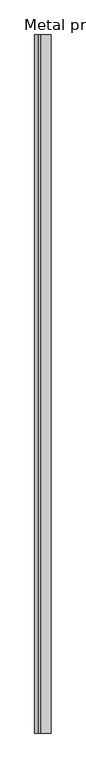
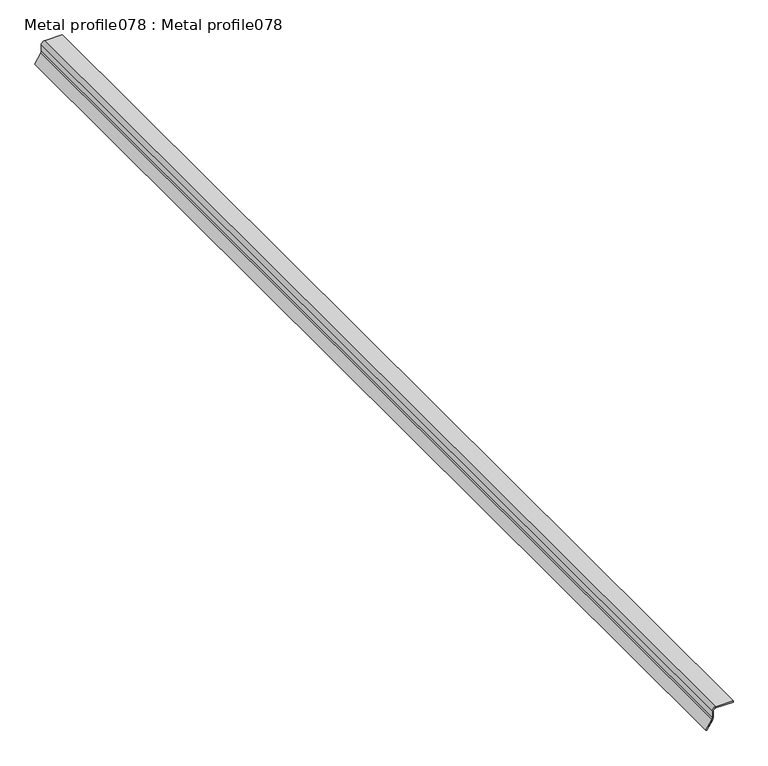
"""IFC4 building model written with IfcOpenShell, lengths in millimetres: proxy geometry, Metal profile078 : Metal profile078."""

from ifc_helpers import new_model, si_unit, point, frame, frame_2d, origin, place, context, project, spatial, polyline, circle_curve, trimmed, segment, composite_curve, outline, extrude, source, transform, mapped, element, save


def metal_profile078_metal_profile078_5d4c4150(model_context):
    return source(origin(), model_context, "Body", "SweptSolid", [
        extrude(outline(composite_curve([segment(polyline([(40166.609375, -9373.5329986), (40168.609375, -9373.5329986), (40168.609375, -9403.2796783)]), True, "CONTINUOUS"), segment(trimmed(circle_curve(frame_2d((40162.259375, -9403.2796783)), 6.35), [point((40168.609375, -9403.2796783))], [point((40162.259375, -9409.6296783))], False, "CARTESIAN"), True, "CONTINUOUS"), segment(polyline([(40162.259375, -9409.6296783), (40151.208717, -9409.6296783)]), True, "CONTINUOUS"), segment(trimmed(circle_curve(frame_2d((40151.208717, -9415.9796783)), 6.35), [point((40151.208717, -9409.6296783))], [point((40147.8972413, -9410.5615025))], True, "CARTESIAN"), True, "CONTINUOUS"), segment(polyline([(40147.8972413, -9410.5615025), (40131.8632813, -9420.3611236), (40130.8202968, -9418.6546115), (40146.8542568, -9408.8549905)]), True, "CONTINUOUS"), segment(trimmed(circle_curve(frame_2d((40151.208717, -9415.9796783)), 8.35), [point((40146.8542568, -9408.8549905))], [point((40151.208717, -9407.6296783))], False, "CARTESIAN"), True, "CONTINUOUS"), segment(polyline([(40151.208717, -9407.6296783), (40162.259375, -9407.6296783)]), True, "CONTINUOUS"), segment(trimmed(circle_curve(frame_2d((40162.259375, -9403.2796783)), 4.35), [point((40162.259375, -9407.6296783))], [point((40166.609375, -9403.2796783))], True, "CARTESIAN"), True, "CONTINUOUS"), segment(polyline([(40166.609375, -9403.2796783), (40166.609375, -9373.5329986)]), True, "CONTINUOUS")], self_intersect=False)), frame((0.0, 7982.1531721, 0.0), z_axis=(0.0, 1.0, 0.0), x_axis=(0.0, 0.0, 1.0)), (0.0, 0.0, 1.0), 2000.0),
    ])


if __name__ == "__main__":
    model = new_model("IFC4")
    model_context = context("Model", 3, world=origin())
    ifc_project = project(units=[si_unit("LENGTHUNIT", "METRE", prefix="MILLI")], contexts=[model_context])
    site = spatial("IfcSite", under=ifc_project)
    building = spatial("IfcBuilding", under=site)
    placement = place(None, origin())
    metal_profile078_metal_profile078_shape = metal_profile078_metal_profile078_5d4c4150(model_context)
    element("IfcBuildingElementProxy", 1, Name="Metal profile078 : Metal profile078", ObjectType="Metal profile078 : Metal profile078", at=placement, inside=building, context=model_context, shape_type="MappedRepresentation", body=[
        mapped(metal_profile078_metal_profile078_shape, transform((0.0, 0.0, 0.0), x_axis=(1.0, 0.0, 0.0), y_axis=(0.0, 1.0, 0.0), z_axis=(0.0, 0.0, 1.0))),
    ])
    save(model, "model.ifc")

# Revit data of these elements
# Type "Metal profile078 : Metal profile078"
#   NameOverride = "Metal profile078"
# Element 1 (IfcBuildingElementProxy, "Metal profile078 : Metal profile078")
#   Materials on its faces: "ANGLE TRIM"
# Materials
#   "ANGLE TRIM": class "Unassigned", colour RGB 250 255 0, transparency 0
